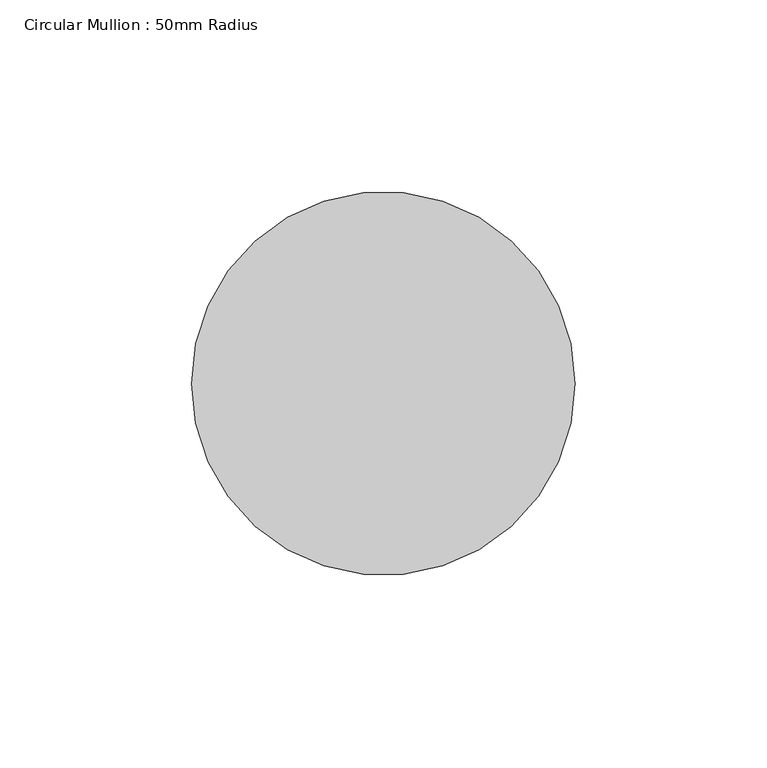
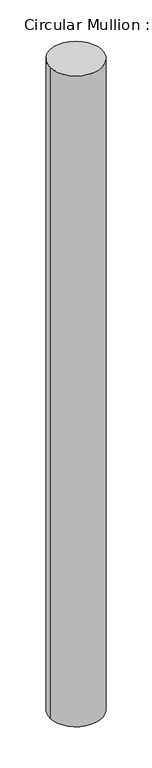
"""IFC4 building model written with IfcOpenShell, lengths in millimetres: member geometry, Circular Mullion : 50mm Radius."""

from ifc_helpers import new_model, si_unit, point, frame, origin, origin_2d, place, context, project, spatial, circle_curve, trimmed, segment, composite_curve, outline, extrude, source, transform, mapped, element, save


def circular_mullion_50mm_radius_18663b67(model_context):
    return source(origin(), model_context, "Body", "SweptSolid", [
        extrude(outline(composite_curve([segment(trimmed(circle_curve(origin_2d(), 50.0), [point((50.0, 0.0))], [point((-50.0, 0.0))], False, "CARTESIAN"), True, "CONTINUOUS"), segment(trimmed(circle_curve(origin_2d(), 50.0), [point((-50.0, 0.0))], [point((50.0, 0.0))], False, "CARTESIAN"), True, "CONTINUOUS")], self_intersect=False)), frame((0.0, 0.0, -1315.2819048), z_axis=(0.0, 0.0, 1.0), x_axis=(1.0, 0.0, 0.0)), (0.0, 0.0, 1.0), 1315.2819048),
    ])


if __name__ == "__main__":
    model = new_model("IFC4")
    model_context = context("Model", 3, world=origin())
    ifc_project = project(units=[si_unit("LENGTHUNIT", "METRE", prefix="MILLI")], contexts=[model_context])
    site = spatial("IfcSite", under=ifc_project)
    building = spatial("IfcBuilding", under=site)
    placement = place(None, origin())
    circular_mullion_50mm_radius_shape = circular_mullion_50mm_radius_18663b67(model_context)
    element("IfcMember", 1, ObjectType="Circular Mullion : 50mm Radius", at=placement, inside=building, context=model_context, shape_type="MappedRepresentation", body=[
        mapped(circular_mullion_50mm_radius_shape, transform((0.0, 0.0, 0.0), x_axis=(1.0, 0.0, 0.0), y_axis=(0.0, 1.0, 0.0), z_axis=(0.0, 0.0, 1.0))),
    ])
    save(model, "model.ifc")

# Revit data of these elements
# Type "Circular Mullion : 50mm Radius"
#   built-in parameter 1007350 = 0.164042 (stored number, unit not read)
# Element 1 (IfcMember, "Circular Mullion : 50mm Radius")
#   Materials on its faces: "Aluminium"
# Materials
#   "Aluminium": class "Metal", colour RGB 247 247 247, transparency 0, Description = "Aluminium 6061", Cost = 0
